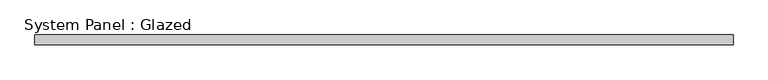
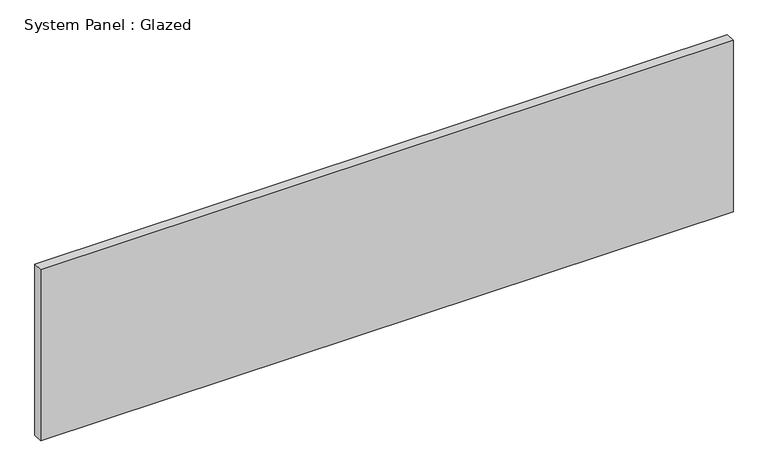
"""IFC4 building model written with IfcOpenShell, lengths in millimetres: plate geometry, System Panel : Glazed."""

from ifc_helpers import new_model, si_unit, origin, origin_with_axes, place, context, project, spatial, polyline, outline, extrude, source, transform, mapped, element, save


def system_panel_glazed_4c2a0bc6(model_context):
    return source(origin(), model_context, "Body", "SweptSolid", [
        extrude(outline(polyline([(890.0000002, 24.5), (-890.0000002, 24.5), (-890.0000002, 49.5), (890.0000002, 49.5), (890.0000002, 24.5)])), origin_with_axes(), (0.0, 0.0, 1.0), 465.0),
    ])


if __name__ == "__main__":
    model = new_model("IFC4")
    model_context = context("Model", 3, world=origin())
    ifc_project = project(units=[si_unit("LENGTHUNIT", "METRE", prefix="MILLI")], contexts=[model_context])
    site = spatial("IfcSite", under=ifc_project)
    building = spatial("IfcBuilding", under=site)
    placement = place(None, origin())
    system_panel_glazed_shape = system_panel_glazed_4c2a0bc6(model_context)
    element("IfcPlate", 1, ObjectType="System Panel : Glazed", at=placement, inside=building, context=model_context, shape_type="MappedRepresentation", body=[
        mapped(system_panel_glazed_shape, transform((0.0, 0.0, 0.0), x_axis=(1.0, 0.0, 0.0), y_axis=(0.0, 1.0, 0.0), z_axis=(0.0, 0.0, 1.0))),
    ])
    save(model, "model.ifc")

# Revit data of these elements
# Element 1 (IfcPlate, "System Panel : Glazed")
#   Materials on its faces: "Glass"
# Materials
#   "Glass": class "Glass", colour RGB 218 227 224, transparency 0.85, Description = "Soda Lime Glass", Cost = 0
